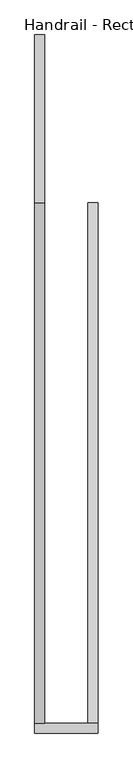
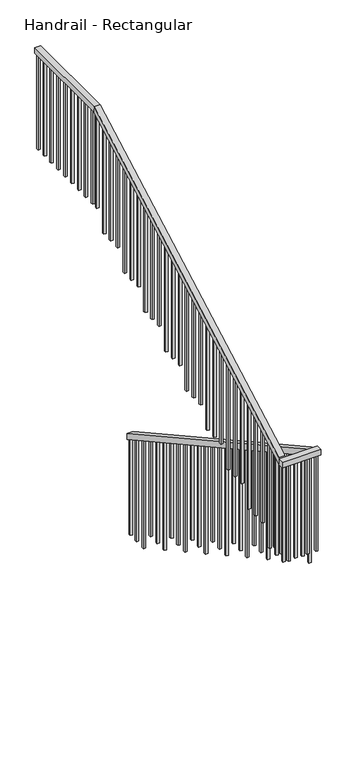
"""IFC4 building model written with IfcOpenShell, lengths in millimetres: railing geometry, Handrail - Rectangular."""

import ifcopenshell
import ifcopenshell.guid

model = None  # the IFC model being written
_history = None  # IfcOwnerHistory: only IFC2X3 demands one
_inside = {}  # id of a spatial element -> (the spatial element, [elements in it])
_under = {}  # id of a project, library or spatial element -> (it, [spatial elements below it])
_declared = {}  # id of a project -> (the project, [libraries it declares])
_typed = {}  # id of a type object -> (the type object, [elements of that type])
_made_of = {}  # id of a material, layer set ... -> (it, [elements and type objects made of it])


def new_model(schema):
    """Start an empty IFC model of exactly this schema.

    Asked for "IFC4X3", IfcOpenShell would pick the latest addendum, in which some entities
    have other attributes; the version numbers below select the first issue.
    IFC2X3 requires an IfcOwnerHistory on every rooted entity: one is made here for all.
    """
    global model, _history
    if schema == "IFC4X3":
        model = ifcopenshell.file(schema_version=(4, 3, 0, 0))
    else:
        model = ifcopenshell.file(schema=schema)
    _inside.clear()
    _under.clear()
    _declared.clear()
    _typed.clear()
    _made_of.clear()
    _history = None
    if model.schema == "IFC2X3":
        org = make("IfcOrganization", Name="unknown")
        user = make(
            "IfcPersonAndOrganization",
            ThePerson=make("IfcPerson", FamilyName="unknown"),
            TheOrganization=org,
        )
        app = make(
            "IfcApplication",
            ApplicationDeveloper=org,
            Version="unknown",
            ApplicationFullName="unknown",
            ApplicationIdentifier="unknown",
        )
        _history = make(
            "IfcOwnerHistory",
            OwningUser=user,
            OwningApplication=app,
            ChangeAction="ADDED",
            CreationDate=0,
        )
    return model


def make(cls, **values):
    """One entity of the class cls with the attributes given. An attribute that is None is left unset."""
    return model.create_entity(
        cls, **{name: value for name, value in values.items() if value is not None}
    )


def rooted(cls, **values):
    """An entity with a GlobalId (a new one), such as an element, a storey or a relation."""
    return make(cls, GlobalId=ifcopenshell.guid.new(), OwnerHistory=_history, **values)


def si_unit(unit_type, name, prefix=None):
    """IfcSIUnit, for example si_unit("LENGTHUNIT", "METRE", prefix="MILLI")."""
    return make("IfcSIUnit", UnitType=unit_type, Prefix=prefix, Name=name)


def assignment(units):
    """IfcUnitAssignment: the units of a project."""
    return None if units is None else make("IfcUnitAssignment", Units=units)


def point(xyz):
    """IfcCartesianPoint."""
    return None if xyz is None else make("IfcCartesianPoint", Coordinates=xyz)


def direction(xyz):
    """IfcDirection."""
    return None if xyz is None else make("IfcDirection", DirectionRatios=xyz)


def frame(location, z_axis=None, x_axis=None):
    """IfcAxis2Placement3D, a coordinate frame: its origin and axes. An axis left out is left unset."""
    return make(
        "IfcAxis2Placement3D",
        Location=point(location),
        Axis=direction(z_axis),
        RefDirection=direction(x_axis),
    )


def origin():
    """The frame at (0, 0, 0) with its axes left unset."""
    return frame((0.0, 0.0, 0.0))


def place(relative_to, where):
    """IfcLocalPlacement: puts the frame where relative to a parent placement (None: the world)."""
    return make(
        "IfcLocalPlacement", PlacementRelTo=relative_to, RelativePlacement=where
    )


def context(
    kind, dimensions, precision=None, world=None, true_north=None, identifier=None
):
    """IfcGeometricRepresentationContext, for example the 3D "Model" context."""
    return make(
        "IfcGeometricRepresentationContext",
        ContextIdentifier=identifier,
        ContextType=kind,
        CoordinateSpaceDimension=dimensions,
        Precision=precision,
        WorldCoordinateSystem=world,
        TrueNorth=true_north,
    )


def project(units=None, contexts=None):
    """IfcProject with its units and contexts."""
    return rooted(
        "IfcProject",
        Name="project",
        RepresentationContexts=contexts,
        UnitsInContext=assignment(units),
    )


def spatial(cls, under=None, at=None, **own):
    """A site, building, storey or space (cls), placed at a placement, below another one or the project."""
    s = rooted(cls, ObjectPlacement=at, **own)
    if under is not None:
        _under.setdefault(under.id(), (under, []))[1].append(s)
    return s


def polyline(points):
    """IfcPolyline through the points."""
    return make("IfcPolyline", Points=[point(p) for p in points])


def outline(outer, holes=None, kind="AREA"):
    """IfcArbitraryClosedProfileDef: a profile drawn as a closed curve; with holes, ...WithVoids."""
    if holes is None:
        return make("IfcArbitraryClosedProfileDef", ProfileType=kind, OuterCurve=outer)
    return make(
        "IfcArbitraryProfileDefWithVoids",
        ProfileType=kind,
        OuterCurve=outer,
        InnerCurves=holes,
    )


def extrude(swept, where, along, depth):
    """IfcExtrudedAreaSolid: the profile swept, set in the frame where, extruded along a direction by depth."""
    return make(
        "IfcExtrudedAreaSolid",
        SweptArea=swept,
        Position=where,
        ExtrudedDirection=direction(along),
        Depth=depth,
    )


def faces_of(points, faces, orient=None, outer=None):
    """IfcFace entities. A face is a list of loops; a loop is a list of indices into points, from 0.

    orient and outer hold one flag for each loop. By default every Orientation is true, the
    first loop of a face is its IfcFaceOuterBound and the others are IfcFaceBound.
    """
    made = []
    for i, loops in enumerate(faces):
        bounds = []
        for j, loop in enumerate(loops):
            is_outer = j == 0 if outer is None else outer[i][j]
            bounds.append(
                make(
                    "IfcFaceOuterBound" if is_outer else "IfcFaceBound",
                    Bound=make("IfcPolyLoop", Polygon=[points[k] for k in loop]),
                    Orientation=True if orient is None else orient[i][j],
                )
            )
        made.append(make("IfcFace", Bounds=bounds))
    return made


def faceted_brep(points, faces, orient=None, outer=None, voids=None):
    """IfcFacetedBrep: a solid bounded by flat faces; with voids (closed shells), ...WithVoids."""
    shared = [point(p) for p in points]
    hull = make("IfcClosedShell", CfsFaces=faces_of(shared, faces, orient, outer))
    if voids is None:
        return make("IfcFacetedBrep", Outer=hull)
    return make(
        "IfcFacetedBrepWithVoids",
        Outer=hull,
        Voids=[
            make(cls, CfsFaces=faces_of(shared, fs, o, b)) for cls, fs, o, b in voids
        ],
    )


def shape(context_of_items, identifier, shape_type, items):
    """IfcShapeRepresentation: the items that make up one representation, for example the "Body"."""
    return make(
        "IfcShapeRepresentation",
        ContextOfItems=context_of_items,
        RepresentationIdentifier=identifier,
        RepresentationType=shape_type,
        Items=items,
    )


def source(mapping_origin, context_of_items, identifier, shape_type, items):
    """IfcRepresentationMap: a shape defined once, which mapped items show again and again."""
    return make(
        "IfcRepresentationMap",
        MappingOrigin=mapping_origin,
        MappedRepresentation=shape(context_of_items, identifier, shape_type, items),
    )


def transform(
    local_origin,
    x_axis=None,
    y_axis=None,
    z_axis=None,
    scale=None,
    scale2=None,
    scale3=None,
    uniform=True,
):
    """IfcCartesianTransformationOperator3D, or its non-uniform kind. x_axis, y_axis, z_axis: its Axis1, 2, 3."""
    if uniform:
        return make(
            "IfcCartesianTransformationOperator3D",
            Axis1=direction(x_axis),
            Axis2=direction(y_axis),
            LocalOrigin=point(local_origin),
            Scale=scale,
            Axis3=direction(z_axis),
        )
    return make(
        "IfcCartesianTransformationOperator3DnonUniform",
        Axis1=direction(x_axis),
        Axis2=direction(y_axis),
        LocalOrigin=point(local_origin),
        Scale=scale,
        Axis3=direction(z_axis),
        Scale2=scale2,
        Scale3=scale3,
    )


def mapped(mapping_source, mapping_target):
    """IfcMappedItem: shows the shape of a source again, moved by a transform."""
    return make(
        "IfcMappedItem", MappingSource=mapping_source, MappingTarget=mapping_target
    )


def made_of(thing, what):
    """Note that an element or type object is made of a material, layer set ...; save() writes the relation."""
    if what is not None:
        _made_of.setdefault(what.id(), (what, []))[1].append(thing)
    return thing


def element(
    cls,
    number,
    at=None,
    inside=None,
    cuts=None,
    type_object=None,
    material=None,
    context=None,
    identifier="Body",
    shape_type=None,
    held_by="IfcProductDefinitionShape",
    body=None,
    shapes=None,
    **own,
):
    """One element of the class cls, such as IfcWall. Its Tag is "e" and its number.

    at: its placement. inside: the storey or other place that contains it. cuts: it is an
    opening in that element (IfcRelVoidsElement). A single representation is given by context,
    identifier, shape_type and body (its items); several are given by shapes. held_by: the class
    of the entity that holds the representations. save() writes the other relations.
    """
    e = rooted(cls, Tag="e%d" % number, ObjectPlacement=at, **own)
    if body is not None:
        shapes = [shape(context, identifier, shape_type, body)]
    if shapes is not None:
        e.Representation = make(held_by, Representations=shapes)
    if inside is not None:
        _inside.setdefault(inside.id(), (inside, []))[1].append(e)
    if cuts is not None:
        rooted(
            "IfcRelVoidsElement", RelatingBuildingElement=cuts, RelatedOpeningElement=e
        )
    if type_object is not None:
        _typed.setdefault(type_object.id(), (type_object, []))[1].append(e)
    return made_of(e, material)


def aggregate(whole, parts):
    """IfcRelAggregates: a whole, such as a stair, and the parts it consists of."""
    return rooted("IfcRelAggregates", RelatingObject=whole, RelatedObjects=parts)


def save(model, path):
    """Write the relations noted so far, then the file.

    IfcRelAggregates (storeys below a building ...), IfcRelContainedInSpatialStructure (elements
    in a storey), IfcRelDefinesByType, IfcRelAssociatesMaterial and IfcRelDeclares: one each for
    every whole, place, type object, material and project.
    """
    for whole, parts in _under.values():
        aggregate(whole, parts)
    for where, things in _inside.values():
        rooted(
            "IfcRelContainedInSpatialStructure",
            RelatedElements=things,
            RelatingStructure=where,
        )
    for kind, things in _typed.values():
        rooted("IfcRelDefinesByType", RelatedObjects=things, RelatingType=kind)
    for what, things in _made_of.values():
        rooted("IfcRelAssociatesMaterial", RelatedObjects=things, RelatingMaterial=what)
    for by, libraries in _declared.values():
        rooted("IfcRelDeclares", RelatingContext=by, RelatedDefinitions=libraries)
    model.write(path)


def handrail_rectangular_766db315(model_context):
    return source(origin(), model_context, "Body", "SolidModel", [
        faceted_brep([(-74723.577375, 13792.2, 13481.05), (-74723.577375, 13792.2, 13430.25), (-74774.377375, 13792.2, 13430.25), (-74774.377375, 13792.2, 13481.05), (-74723.577375, 12915.9, 13481.05), (-74723.577375, 12929.0029811, 13430.25), (-74774.377375, 12929.0029811, 13430.25), (-74774.377375, 12915.9, 13481.05), (-74723.577375, 10198.1, 11979.1078947), (-74774.377375, 10198.1, 11979.1078947), (-74774.377375, 10198.1, 11921.0667736), (-74723.577375, 10198.1, 11921.0667736)], [[[0, 1, 2, 3]], [[1, 0, 4, 5]], [[2, 1, 5, 6]], [[3, 2, 6, 7]], [[0, 3, 7, 4]], [[8, 9, 10, 11]], [[5, 4, 8, 11]], [[6, 5, 11, 10]], [[7, 6, 10, 9]], [[4, 7, 9, 8]]]),
        faceted_brep([(-74774.377375, 10198.1, 11965.0710526), (-74774.377375, 10198.1, 11914.2710526), (-74774.377375, 10147.3, 11914.2710526), (-74774.377375, 10147.3, 11965.0710526), (-74444.177375, 10198.1, 11965.0710526), (-74444.177375, 10147.3, 11965.0710526), (-74444.177375, 10147.3, 11914.2710526), (-74444.177375, 10198.1, 11914.2710526)], [[[0, 1, 2, 3]], [[4, 5, 6, 7]], [[1, 0, 4, 7]], [[2, 1, 7, 6]], [[3, 2, 6, 5]], [[0, 3, 5, 4]]]),
        faceted_brep([(-74494.977375, 10198.1, 11951.0342105), (-74494.977375, 10198.1, 11892.9930894), (-74444.177375, 10198.1, 11892.9930894), (-74444.177375, 10198.1, 11951.0342105), (-74494.977375, 12915.9, 10449.0921053), (-74444.177375, 12915.9, 10449.0921053), (-74444.177375, 12915.9, 10391.0509841), (-74494.977375, 12915.9, 10391.0509841)], [[[0, 1, 2, 3]], [[4, 5, 6, 7]], [[1, 0, 4, 7]], [[2, 1, 7, 6]], [[3, 2, 6, 5]], [[0, 3, 5, 4]]]),
        extrude(outline(polyline([(12823.825, 10441.9345367), (12823.825, 9534.6921053), (12804.775, 9534.6921053), (12804.775, 10452.4621683), (12823.825, 10441.9345367)])), frame((-74479.102375, 0.0, 0.0), z_axis=(1.0, 0.0, 0.0), x_axis=(0.0, 1.0, 0.0)), (0.0, 0.0, 1.0), 19.05),
        extrude(outline(polyline([(12722.225, 10498.0819052), (12722.225, 9534.6921053), (12703.175, 9534.6921053), (12703.175, 10508.6095367), (12722.225, 10498.0819052)])), frame((-74479.102375, 0.0, 0.0), z_axis=(1.0, 0.0, 0.0), x_axis=(0.0, 1.0, 0.0)), (0.0, 0.0, 1.0), 19.05),
        extrude(outline(polyline([(12620.625, 10554.2292736), (12620.625, 9703.1342105), (12601.575, 9703.1342105), (12601.575, 10564.7569052), (12620.625, 10554.2292736)])), frame((-74479.102375, 0.0, 0.0), z_axis=(1.0, 0.0, 0.0), x_axis=(0.0, 1.0, 0.0)), (0.0, 0.0, 1.0), 19.05),
        extrude(outline(polyline([(12519.025, 10610.376642), (12519.025, 9703.1342105), (12499.975, 9703.1342105), (12499.975, 10620.9042736), (12519.025, 10610.376642)])), frame((-74479.102375, 0.0, 0.0), z_axis=(1.0, 0.0, 0.0), x_axis=(0.0, 1.0, 0.0)), (0.0, 0.0, 1.0), 19.05),
        extrude(outline(polyline([(12417.425, 10666.5240104), (12417.425, 9703.1342105), (12398.375, 9703.1342105), (12398.375, 10677.051642), (12417.425, 10666.5240104)])), frame((-74479.102375, 0.0, 0.0), z_axis=(1.0, 0.0, 0.0), x_axis=(0.0, 1.0, 0.0)), (0.0, 0.0, 1.0), 19.05),
        extrude(outline(polyline([(12315.825, 10722.6713788), (12315.825, 9871.5763158), (12296.775, 9871.5763158), (12296.775, 10733.1990104), (12315.825, 10722.6713788)])), frame((-74479.102375, 0.0, 0.0), z_axis=(1.0, 0.0, 0.0), x_axis=(0.0, 1.0, 0.0)), (0.0, 0.0, 1.0), 19.05),
        extrude(outline(polyline([(12214.225, 10778.8187473), (12214.225, 9871.5763158), (12195.175, 9871.5763158), (12195.175, 10789.3463788), (12214.225, 10778.8187473)])), frame((-74479.102375, 0.0, 0.0), z_axis=(1.0, 0.0, 0.0), x_axis=(0.0, 1.0, 0.0)), (0.0, 0.0, 1.0), 19.05),
        extrude(outline(polyline([(12112.625, 10834.9661157), (12112.625, 9871.5763158), (12093.575, 9871.5763158), (12093.575, 10845.4937473), (12112.625, 10834.9661157)])), frame((-74479.102375, 0.0, 0.0), z_axis=(1.0, 0.0, 0.0), x_axis=(0.0, 1.0, 0.0)), (0.0, 0.0, 1.0), 19.05),
        extrude(outline(polyline([(12011.025, 10891.1134841), (12011.025, 10040.0184211), (11991.975, 10040.0184211), (11991.975, 10901.6411157), (12011.025, 10891.1134841)])), frame((-74479.102375, 0.0, 0.0), z_axis=(1.0, 0.0, 0.0), x_axis=(0.0, 1.0, 0.0)), (0.0, 0.0, 1.0), 19.05),
        extrude(outline(polyline([(11909.425, 10947.2608525), (11909.425, 10040.0184211), (11890.375, 10040.0184211), (11890.375, 10957.7884841), (11909.425, 10947.2608525)])), frame((-74479.102375, 0.0, 0.0), z_axis=(1.0, 0.0, 0.0), x_axis=(0.0, 1.0, 0.0)), (0.0, 0.0, 1.0), 19.05),
        extrude(outline(polyline([(11807.825, 11003.4082209), (11807.825, 10040.0184211), (11788.775, 10040.0184211), (11788.775, 11013.9358525), (11807.825, 11003.4082209)])), frame((-74479.102375, 0.0, 0.0), z_axis=(1.0, 0.0, 0.0), x_axis=(0.0, 1.0, 0.0)), (0.0, 0.0, 1.0), 19.05),
        extrude(outline(polyline([(11706.225, 11059.5555894), (11706.225, 10208.4605263), (11687.175, 10208.4605263), (11687.175, 11070.0832209), (11706.225, 11059.5555894)])), frame((-74479.102375, 0.0, 0.0), z_axis=(1.0, 0.0, 0.0), x_axis=(0.0, 1.0, 0.0)), (0.0, 0.0, 1.0), 19.05),
        extrude(outline(polyline([(11604.625, 11115.7029578), (11604.625, 10208.4605263), (11585.575, 10208.4605263), (11585.575, 11126.2305894), (11604.625, 11115.7029578)])), frame((-74479.102375, 0.0, 0.0), z_axis=(1.0, 0.0, 0.0), x_axis=(0.0, 1.0, 0.0)), (0.0, 0.0, 1.0), 19.05),
        extrude(outline(polyline([(11503.025, 11171.8503262), (11503.025, 10208.4605263), (11483.975, 10208.4605263), (11483.975, 11182.3779578), (11503.025, 11171.8503262)])), frame((-74479.102375, 0.0, 0.0), z_axis=(1.0, 0.0, 0.0), x_axis=(0.0, 1.0, 0.0)), (0.0, 0.0, 1.0), 19.05),
        extrude(outline(polyline([(11401.425, 11227.9976946), (11401.425, 10376.9026316), (11382.375, 10376.9026316), (11382.375, 11238.5253262), (11401.425, 11227.9976946)])), frame((-74479.102375, 0.0, 0.0), z_axis=(1.0, 0.0, 0.0), x_axis=(0.0, 1.0, 0.0)), (0.0, 0.0, 1.0), 19.05),
        extrude(outline(polyline([(11299.825, 11284.1450631), (11299.825, 10376.9026316), (11280.775, 10376.9026316), (11280.775, 11294.6726946), (11299.825, 11284.1450631)])), frame((-74479.102375, 0.0, 0.0), z_axis=(1.0, 0.0, 0.0), x_axis=(0.0, 1.0, 0.0)), (0.0, 0.0, 1.0), 19.05),
        extrude(outline(polyline([(11198.225, 11340.2924315), (11198.225, 10376.9026316), (11179.175, 10376.9026316), (11179.175, 11350.8200631), (11198.225, 11340.2924315)])), frame((-74479.102375, 0.0, 0.0), z_axis=(1.0, 0.0, 0.0), x_axis=(0.0, 1.0, 0.0)), (0.0, 0.0, 1.0), 19.05),
        extrude(outline(polyline([(11096.625, 11396.4397999), (11096.625, 10545.3447368), (11077.575, 10545.3447368), (11077.575, 11406.9674315), (11096.625, 11396.4397999)])), frame((-74479.102375, 0.0, 0.0), z_axis=(1.0, 0.0, 0.0), x_axis=(0.0, 1.0, 0.0)), (0.0, 0.0, 1.0), 19.05),
        extrude(outline(polyline([(10995.025, 11452.5871683), (10995.025, 10545.3447368), (10975.975, 10545.3447368), (10975.975, 11463.1147999), (10995.025, 11452.5871683)])), frame((-74479.102375, 0.0, 0.0), z_axis=(1.0, 0.0, 0.0), x_axis=(0.0, 1.0, 0.0)), (0.0, 0.0, 1.0), 19.05),
        extrude(outline(polyline([(10893.425, 11508.7345367), (10893.425, 10545.3447368), (10874.375, 10545.3447368), (10874.375, 11519.2621683), (10893.425, 11508.7345367)])), frame((-74479.102375, 0.0, 0.0), z_axis=(1.0, 0.0, 0.0), x_axis=(0.0, 1.0, 0.0)), (0.0, 0.0, 1.0), 19.05),
        extrude(outline(polyline([(10791.825, 11564.8819052), (10791.825, 10713.7868421), (10772.775, 10713.7868421), (10772.775, 11575.4095367), (10791.825, 11564.8819052)])), frame((-74479.102375, 0.0, 0.0), z_axis=(1.0, 0.0, 0.0), x_axis=(0.0, 1.0, 0.0)), (0.0, 0.0, 1.0), 19.05),
        extrude(outline(polyline([(10690.225, 11621.0292736), (10690.225, 10713.7868421), (10671.175, 10713.7868421), (10671.175, 11631.5569052), (10690.225, 11621.0292736)])), frame((-74479.102375, 0.0, 0.0), z_axis=(1.0, 0.0, 0.0), x_axis=(0.0, 1.0, 0.0)), (0.0, 0.0, 1.0), 19.05),
        extrude(outline(polyline([(10588.625, 11677.176642), (10588.625, 10713.7868421), (10569.575, 10713.7868421), (10569.575, 11687.7042736), (10588.625, 11677.176642)])), frame((-74479.102375, 0.0, 0.0), z_axis=(1.0, 0.0, 0.0), x_axis=(0.0, 1.0, 0.0)), (0.0, 0.0, 1.0), 19.05),
        extrude(outline(polyline([(10487.025, 11733.3240104), (10487.025, 10882.2289474), (10467.975, 10882.2289474), (10467.975, 11743.851642), (10487.025, 11733.3240104)])), frame((-74479.102375, 0.0, 0.0), z_axis=(1.0, 0.0, 0.0), x_axis=(0.0, 1.0, 0.0)), (0.0, 0.0, 1.0), 19.05),
        extrude(outline(polyline([(10385.425, 11789.4713788), (10385.425, 10882.2289474), (10366.375, 10882.2289474), (10366.375, 11799.9990104), (10385.425, 11789.4713788)])), frame((-74479.102375, 0.0, 0.0), z_axis=(1.0, 0.0, 0.0), x_axis=(0.0, 1.0, 0.0)), (0.0, 0.0, 1.0), 19.05),
        extrude(outline(polyline([(10283.825, 11845.6187473), (10283.825, 10882.2289474), (10264.775, 10882.2289474), (10264.775, 11856.1463788), (10283.825, 11845.6187473)])), frame((-74479.102375, 0.0, 0.0), z_axis=(1.0, 0.0, 0.0), x_axis=(0.0, 1.0, 0.0)), (0.0, 0.0, 1.0), 19.05),
        extrude(outline(polyline([(-74555.302375, 10182.225), (-74536.252375, 10182.225), (-74536.252375, 10163.175), (-74555.302375, 10163.175), (-74555.302375, 10182.225)])), frame((0.0, 0.0, 11050.6710526), z_axis=(0.0, 0.0, 1.0), x_axis=(1.0, 0.0, 0.0)), (0.0, 0.0, 1.0), 863.6),
        extrude(outline(polyline([(-74656.902375, 10182.225), (-74637.852375, 10182.225), (-74637.852375, 10163.175), (-74656.902375, 10163.175), (-74656.902375, 10182.225)])), frame((0.0, 0.0, 11050.6710526), z_axis=(0.0, 0.0, 1.0), x_axis=(1.0, 0.0, 0.0)), (0.0, 0.0, 1.0), 863.6),
        extrude(outline(polyline([(10283.825, 11968.4411157), (10283.825, 11050.6710526), (10264.775, 11050.6710526), (10264.775, 11957.9134841), (10283.825, 11968.4411157)])), frame((-74758.502375, 0.0, 0.0), z_axis=(1.0, 0.0, 0.0), x_axis=(0.0, 1.0, 0.0)), (0.0, 0.0, 1.0), 19.05),
        extrude(outline(polyline([(10385.425, 12024.5884841), (10385.425, 11050.6710526), (10366.375, 11050.6710526), (10366.375, 12014.0608525), (10385.425, 12024.5884841)])), frame((-74758.502375, 0.0, 0.0), z_axis=(1.0, 0.0, 0.0), x_axis=(0.0, 1.0, 0.0)), (0.0, 0.0, 1.0), 19.05),
        extrude(outline(polyline([(10487.025, 12080.7358525), (10487.025, 11219.1131579), (10467.975, 11219.1131579), (10467.975, 12070.2082209), (10487.025, 12080.7358525)])), frame((-74758.502375, 0.0, 0.0), z_axis=(1.0, 0.0, 0.0), x_axis=(0.0, 1.0, 0.0)), (0.0, 0.0, 1.0), 19.05),
        extrude(outline(polyline([(10588.625, 12136.8832209), (10588.625, 11219.1131579), (10569.575, 11219.1131579), (10569.575, 12126.3555894), (10588.625, 12136.8832209)])), frame((-74758.502375, 0.0, 0.0), z_axis=(1.0, 0.0, 0.0), x_axis=(0.0, 1.0, 0.0)), (0.0, 0.0, 1.0), 19.05),
        extrude(outline(polyline([(10690.225, 12193.0305894), (10690.225, 11219.1131579), (10671.175, 11219.1131579), (10671.175, 12182.5029578), (10690.225, 12193.0305894)])), frame((-74758.502375, 0.0, 0.0), z_axis=(1.0, 0.0, 0.0), x_axis=(0.0, 1.0, 0.0)), (0.0, 0.0, 1.0), 19.05),
        extrude(outline(polyline([(10791.825, 12249.1779578), (10791.825, 11387.5552632), (10772.775, 11387.5552632), (10772.775, 12238.6503262), (10791.825, 12249.1779578)])), frame((-74758.502375, 0.0, 0.0), z_axis=(1.0, 0.0, 0.0), x_axis=(0.0, 1.0, 0.0)), (0.0, 0.0, 1.0), 19.05),
        extrude(outline(polyline([(10893.425, 12305.3253262), (10893.425, 11387.5552632), (10874.375, 11387.5552632), (10874.375, 12294.7976946), (10893.425, 12305.3253262)])), frame((-74758.502375, 0.0, 0.0), z_axis=(1.0, 0.0, 0.0), x_axis=(0.0, 1.0, 0.0)), (0.0, 0.0, 1.0), 19.05),
        extrude(outline(polyline([(10995.025, 12361.4726946), (10995.025, 11387.5552632), (10975.975, 11387.5552632), (10975.975, 12350.9450631), (10995.025, 12361.4726946)])), frame((-74758.502375, 0.0, 0.0), z_axis=(1.0, 0.0, 0.0), x_axis=(0.0, 1.0, 0.0)), (0.0, 0.0, 1.0), 19.05),
        extrude(outline(polyline([(11096.625, 12417.6200631), (11096.625, 11555.9973684), (11077.575, 11555.9973684), (11077.575, 12407.0924315), (11096.625, 12417.6200631)])), frame((-74758.502375, 0.0, 0.0), z_axis=(1.0, 0.0, 0.0), x_axis=(0.0, 1.0, 0.0)), (0.0, 0.0, 1.0), 19.05),
        extrude(outline(polyline([(11198.225, 12473.7674315), (11198.225, 11555.9973684), (11179.175, 11555.9973684), (11179.175, 12463.2397999), (11198.225, 12473.7674315)])), frame((-74758.502375, 0.0, 0.0), z_axis=(1.0, 0.0, 0.0), x_axis=(0.0, 1.0, 0.0)), (0.0, 0.0, 1.0), 19.05),
        extrude(outline(polyline([(11299.825, 12529.9147999), (11299.825, 11555.9973684), (11280.775, 11555.9973684), (11280.775, 12519.3871683), (11299.825, 12529.9147999)])), frame((-74758.502375, 0.0, 0.0), z_axis=(1.0, 0.0, 0.0), x_axis=(0.0, 1.0, 0.0)), (0.0, 0.0, 1.0), 19.05),
        extrude(outline(polyline([(11401.425, 12586.0621683), (11401.425, 11724.4394737), (11382.375, 11724.4394737), (11382.375, 12575.5345367), (11401.425, 12586.0621683)])), frame((-74758.502375, 0.0, 0.0), z_axis=(1.0, 0.0, 0.0), x_axis=(0.0, 1.0, 0.0)), (0.0, 0.0, 1.0), 19.05),
        extrude(outline(polyline([(11503.025, 12642.2095367), (11503.025, 11724.4394737), (11483.975, 11724.4394737), (11483.975, 12631.6819052), (11503.025, 12642.2095367)])), frame((-74758.502375, 0.0, 0.0), z_axis=(1.0, 0.0, 0.0), x_axis=(0.0, 1.0, 0.0)), (0.0, 0.0, 1.0), 19.05),
        extrude(outline(polyline([(11604.625, 12698.3569052), (11604.625, 11724.4394737), (11585.575, 11724.4394737), (11585.575, 12687.8292736), (11604.625, 12698.3569052)])), frame((-74758.502375, 0.0, 0.0), z_axis=(1.0, 0.0, 0.0), x_axis=(0.0, 1.0, 0.0)), (0.0, 0.0, 1.0), 19.05),
        extrude(outline(polyline([(11706.225, 12754.5042736), (11706.225, 11892.8815789), (11687.175, 11892.8815789), (11687.175, 12743.976642), (11706.225, 12754.5042736)])), frame((-74758.502375, 0.0, 0.0), z_axis=(1.0, 0.0, 0.0), x_axis=(0.0, 1.0, 0.0)), (0.0, 0.0, 1.0), 19.05),
        extrude(outline(polyline([(11807.825, 12810.651642), (11807.825, 11892.8815789), (11788.775, 11892.8815789), (11788.775, 12800.1240104), (11807.825, 12810.651642)])), frame((-74758.502375, 0.0, 0.0), z_axis=(1.0, 0.0, 0.0), x_axis=(0.0, 1.0, 0.0)), (0.0, 0.0, 1.0), 19.05),
        extrude(outline(polyline([(11909.425, 12866.7990104), (11909.425, 11892.8815789), (11890.375, 11892.8815789), (11890.375, 12856.2713788), (11909.425, 12866.7990104)])), frame((-74758.502375, 0.0, 0.0), z_axis=(1.0, 0.0, 0.0), x_axis=(0.0, 1.0, 0.0)), (0.0, 0.0, 1.0), 19.05),
        extrude(outline(polyline([(12011.025, 12922.9463788), (12011.025, 12061.3236842), (11991.975, 12061.3236842), (11991.975, 12912.4187473), (12011.025, 12922.9463788)])), frame((-74758.502375, 0.0, 0.0), z_axis=(1.0, 0.0, 0.0), x_axis=(0.0, 1.0, 0.0)), (0.0, 0.0, 1.0), 19.05),
        extrude(outline(polyline([(12112.625, 12979.0937473), (12112.625, 12061.3236842), (12093.575, 12061.3236842), (12093.575, 12968.5661157), (12112.625, 12979.0937473)])), frame((-74758.502375, 0.0, 0.0), z_axis=(1.0, 0.0, 0.0), x_axis=(0.0, 1.0, 0.0)), (0.0, 0.0, 1.0), 19.05),
        extrude(outline(polyline([(12214.225, 13035.2411157), (12214.225, 12061.3236842), (12195.175, 12061.3236842), (12195.175, 13024.7134841), (12214.225, 13035.2411157)])), frame((-74758.502375, 0.0, 0.0), z_axis=(1.0, 0.0, 0.0), x_axis=(0.0, 1.0, 0.0)), (0.0, 0.0, 1.0), 19.05),
        extrude(outline(polyline([(12315.825, 13091.3884841), (12315.825, 12229.7657895), (12296.775, 12229.7657895), (12296.775, 13080.8608525), (12315.825, 13091.3884841)])), frame((-74758.502375, 0.0, 0.0), z_axis=(1.0, 0.0, 0.0), x_axis=(0.0, 1.0, 0.0)), (0.0, 0.0, 1.0), 19.05),
        extrude(outline(polyline([(12417.425, 13147.5358525), (12417.425, 12229.7657895), (12398.375, 12229.7657895), (12398.375, 13137.0082209), (12417.425, 13147.5358525)])), frame((-74758.502375, 0.0, 0.0), z_axis=(1.0, 0.0, 0.0), x_axis=(0.0, 1.0, 0.0)), (0.0, 0.0, 1.0), 19.05),
        extrude(outline(polyline([(12519.025, 13203.6832209), (12519.025, 12229.7657895), (12499.975, 12229.7657895), (12499.975, 13193.1555894), (12519.025, 13203.6832209)])), frame((-74758.502375, 0.0, 0.0), z_axis=(1.0, 0.0, 0.0), x_axis=(0.0, 1.0, 0.0)), (0.0, 0.0, 1.0), 19.05),
        extrude(outline(polyline([(12620.625, 13259.8305894), (12620.625, 12398.2078947), (12601.575, 12398.2078947), (12601.575, 13249.3029578), (12620.625, 13259.8305894)])), frame((-74758.502375, 0.0, 0.0), z_axis=(1.0, 0.0, 0.0), x_axis=(0.0, 1.0, 0.0)), (0.0, 0.0, 1.0), 19.05),
        extrude(outline(polyline([(12722.225, 13315.9779578), (12722.225, 12398.2078947), (12703.175, 12398.2078947), (12703.175, 13305.4503262), (12722.225, 13315.9779578)])), frame((-74758.502375, 0.0, 0.0), z_axis=(1.0, 0.0, 0.0), x_axis=(0.0, 1.0, 0.0)), (0.0, 0.0, 1.0), 19.05),
        extrude(outline(polyline([(12823.825, 13372.1253262), (12823.825, 12398.2078947), (12804.775, 12398.2078947), (12804.775, 13361.5976946), (12823.825, 13372.1253262)])), frame((-74758.502375, 0.0, 0.0), z_axis=(1.0, 0.0, 0.0), x_axis=(0.0, 1.0, 0.0)), (0.0, 0.0, 1.0), 19.05),
        extrude(outline(polyline([(-74739.452375, 12988.925), (-74739.452375, 12969.875), (-74758.502375, 12969.875), (-74758.502375, 12988.925), (-74739.452375, 12988.925)])), frame((0.0, 0.0, 12566.65), z_axis=(0.0, 0.0, 1.0), x_axis=(1.0, 0.0, 0.0)), (0.0, 0.0, 1.0), 863.6),
        extrude(outline(polyline([(-74739.452375, 13090.525), (-74739.452375, 13071.475), (-74758.502375, 13071.475), (-74758.502375, 13090.525), (-74739.452375, 13090.525)])), frame((0.0, 0.0, 12566.65), z_axis=(0.0, 0.0, 1.0), x_axis=(1.0, 0.0, 0.0)), (0.0, 0.0, 1.0), 863.6),
        extrude(outline(polyline([(-74739.452375, 13192.125), (-74739.452375, 13173.075), (-74758.502375, 13173.075), (-74758.502375, 13192.125), (-74739.452375, 13192.125)])), frame((0.0, 0.0, 12566.65), z_axis=(0.0, 0.0, 1.0), x_axis=(1.0, 0.0, 0.0)), (0.0, 0.0, 1.0), 863.6),
        extrude(outline(polyline([(-74739.452375, 13293.725), (-74739.452375, 13274.675), (-74758.502375, 13274.675), (-74758.502375, 13293.725), (-74739.452375, 13293.725)])), frame((0.0, 0.0, 12566.65), z_axis=(0.0, 0.0, 1.0), x_axis=(1.0, 0.0, 0.0)), (0.0, 0.0, 1.0), 863.6),
        extrude(outline(polyline([(-74739.452375, 13395.325), (-74739.452375, 13376.275), (-74758.502375, 13376.275), (-74758.502375, 13395.325), (-74739.452375, 13395.325)])), frame((0.0, 0.0, 12566.65), z_axis=(0.0, 0.0, 1.0), x_axis=(1.0, 0.0, 0.0)), (0.0, 0.0, 1.0), 863.6),
        extrude(outline(polyline([(-74739.452375, 13496.925), (-74739.452375, 13477.875), (-74758.502375, 13477.875), (-74758.502375, 13496.925), (-74739.452375, 13496.925)])), frame((0.0, 0.0, 12566.65), z_axis=(0.0, 0.0, 1.0), x_axis=(1.0, 0.0, 0.0)), (0.0, 0.0, 1.0), 863.6),
        extrude(outline(polyline([(-74739.452375, 13598.525), (-74739.452375, 13579.475), (-74758.502375, 13579.475), (-74758.502375, 13598.525), (-74739.452375, 13598.525)])), frame((0.0, 0.0, 12566.65), z_axis=(0.0, 0.0, 1.0), x_axis=(1.0, 0.0, 0.0)), (0.0, 0.0, 1.0), 863.6),
        extrude(outline(polyline([(-74739.452375, 13700.125), (-74739.452375, 13681.075), (-74758.502375, 13681.075), (-74758.502375, 13700.125), (-74739.452375, 13700.125)])), frame((0.0, 0.0, 12566.65), z_axis=(0.0, 0.0, 1.0), x_axis=(1.0, 0.0, 0.0)), (0.0, 0.0, 1.0), 863.6),
        extrude(outline(polyline([(-74479.102375, 10182.225), (-74460.052375, 10182.225), (-74460.052375, 10163.175), (-74479.102375, 10163.175), (-74479.102375, 10182.225)])), frame((0.0, 0.0, 11050.6710526), z_axis=(0.0, 0.0, 1.0), x_axis=(1.0, 0.0, 0.0)), (0.0, 0.0, 1.0), 863.6),
        extrude(outline(polyline([(10182.225, 11912.2937473), (10182.225, 11050.6710526), (10163.175, 11050.6710526), (10163.175, 11901.7661157), (10182.225, 11912.2937473)])), frame((-74758.502375, 0.0, 0.0), z_axis=(1.0, 0.0, 0.0), x_axis=(0.0, 1.0, 0.0)), (0.0, 0.0, 1.0), 19.05),
        extrude(outline(polyline([(-74739.452375, 12925.425), (-74739.452375, 12906.375), (-74758.502375, 12906.375), (-74758.502375, 12925.425), (-74739.452375, 12925.425)])), frame((0.0, 0.0, 12566.65), z_axis=(0.0, 0.0, 1.0), x_axis=(1.0, 0.0, 0.0)), (0.0, 0.0, 1.0), 863.6),
        extrude(outline(polyline([(12915.9, 10391.0509841), (12915.9, 9534.6921053), (12896.85, 9534.6921053), (12896.85, 10401.5786157), (12915.9, 10391.0509841)])), frame((-74479.102375, 0.0, 0.0), z_axis=(1.0, 0.0, 0.0), x_axis=(0.0, 1.0, 0.0)), (0.0, 0.0, 1.0), 19.05),
        extrude(outline(polyline([(-74739.452375, 13792.2), (-74739.452375, 13773.15), (-74758.502375, 13773.15), (-74758.502375, 13792.2), (-74739.452375, 13792.2)])), frame((0.0, 0.0, 12566.65), z_axis=(0.0, 0.0, 1.0), x_axis=(1.0, 0.0, 0.0)), (0.0, 0.0, 1.0), 863.6),
    ])


if __name__ == "__main__":
    model = new_model("IFC4")
    model_context = context("Model", 3, world=origin())
    ifc_project = project(units=[si_unit("LENGTHUNIT", "METRE", prefix="MILLI")], contexts=[model_context])
    site = spatial("IfcSite", under=ifc_project)
    building = spatial("IfcBuilding", under=site)
    placement = place(None, origin())
    handrail_rectangular_shape = handrail_rectangular_766db315(model_context)
    element("IfcRailing", 1, ObjectType="Handrail - Rectangular", at=placement, inside=building, context=model_context, shape_type="MappedRepresentation", body=[
        mapped(handrail_rectangular_shape, transform((0.0, 0.0, 0.0), x_axis=(1.0, 0.0, 0.0), y_axis=(0.0, 1.0, 0.0), z_axis=(0.0, 0.0, 1.0))),
    ])
    save(model, "model.ifc")
